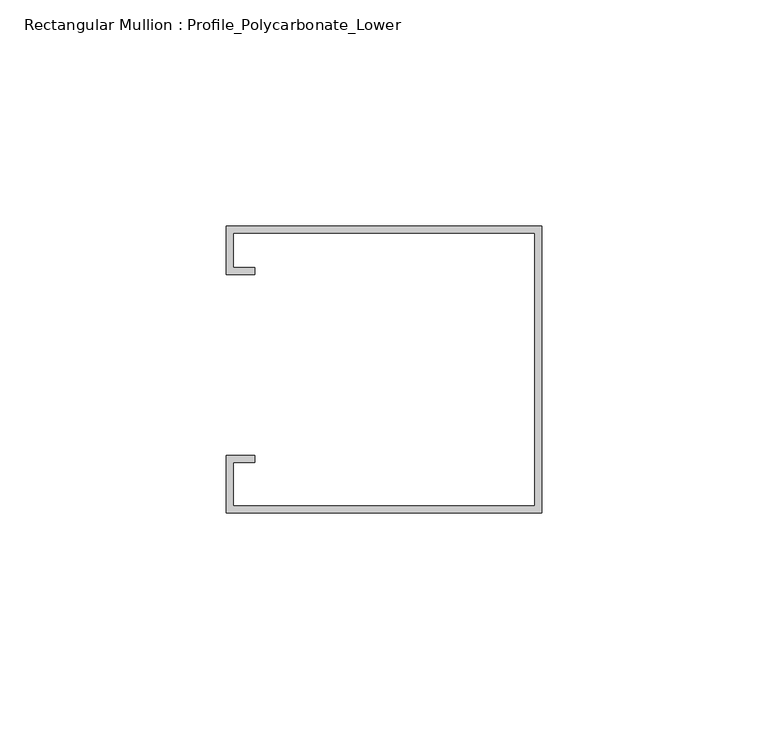
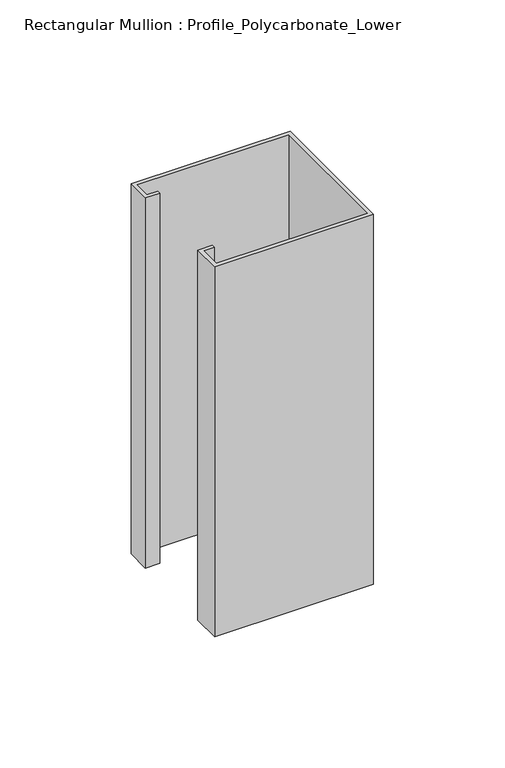
"""IFC4 building model written with IfcOpenShell, lengths in millimetres: member geometry, Rectangular Mullion : Profile_Polycarbonate_Lower."""

from ifc_helpers import new_model, si_unit, frame, origin, place, context, project, spatial, polyline, outline, extrude, source, transform, mapped, element, save


def rectangular_mullion_profile_polycarbonate_lower_6c9cb654(model_context):
    return source(origin(), model_context, "Body", "SweptSolid", [
        extrude(outline(polyline([(0.0, -32.7), (-69.85, -32.7), (-69.85, -20.0), (-63.5, -20.0), (-63.5, -21.5875), (-68.2625, -21.5875), (-68.2625, -31.1125), (-1.5875, -31.1125), (-1.5875, 29.2125), (-68.2625, 29.2125), (-68.2625, 21.5875), (-63.5, 21.5875), (-63.5, 20.0), (-69.85, 20.0), (-69.85, 30.8), (0.0, 30.8), (0.0, -32.7)])), frame((0.0, 0.0, -172.1185239), z_axis=(0.0, 0.0, 1.0), x_axis=(1.0, 0.0, 0.0)), (0.0, 0.0, 1.0), 172.1185239),
    ])


if __name__ == "__main__":
    model = new_model("IFC4")
    model_context = context("Model", 3, world=origin())
    ifc_project = project(units=[si_unit("LENGTHUNIT", "METRE", prefix="MILLI")], contexts=[model_context])
    site = spatial("IfcSite", under=ifc_project)
    building = spatial("IfcBuilding", under=site)
    placement = place(None, origin())
    rectangular_mullion_profile_polycarbonate_lower_shape = rectangular_mullion_profile_polycarbonate_lower_6c9cb654(model_context)
    element("IfcMember", 1, ObjectType="Rectangular Mullion : Profile_Polycarbonate_Lower", at=placement, inside=building, context=model_context, shape_type="MappedRepresentation", body=[
        mapped(rectangular_mullion_profile_polycarbonate_lower_shape, transform((0.0, 0.0, 0.0), x_axis=(1.0, 0.0, 0.0), y_axis=(0.0, 1.0, 0.0), z_axis=(0.0, 0.0, 1.0))),
    ])
    save(model, "model.ifc")

# Revit data of these elements
# Type "Rectangular Mullion : Profile_Polycarbonate_Lower"
#   built-in parameter 1007322 = 0.208333 (stored number, unit not read)
#   built-in parameter 1007321 = 0 (stored number, unit not read)
#   built-in parameter 1007320 = 0.00520833 (stored number, unit not read)
# Element 1 (IfcMember, "Rectangular Mullion : Profile_Polycarbonate_Lower")
#   Materials on its faces: "GALVANIZED UNISTRUT P5500, 1 5/8\" X 2 7/16\" OR ALUM. CHANNEL"
# Materials
#   "GALVANIZED UNISTRUT P5500, 1 5/8\" X 2 7/16\" OR ALUM. CHANNEL": class "Metal", colour RGB 244 244 244, transparency 0, Description = "Aluminum 6061", Cost = 0
